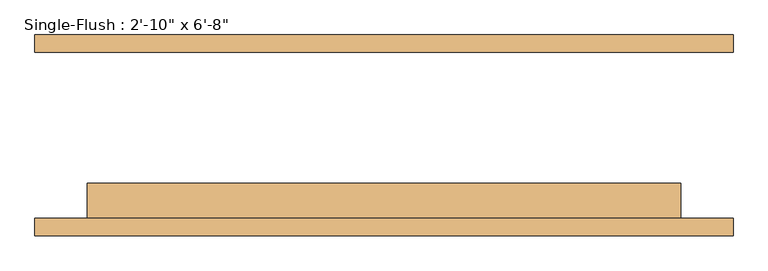
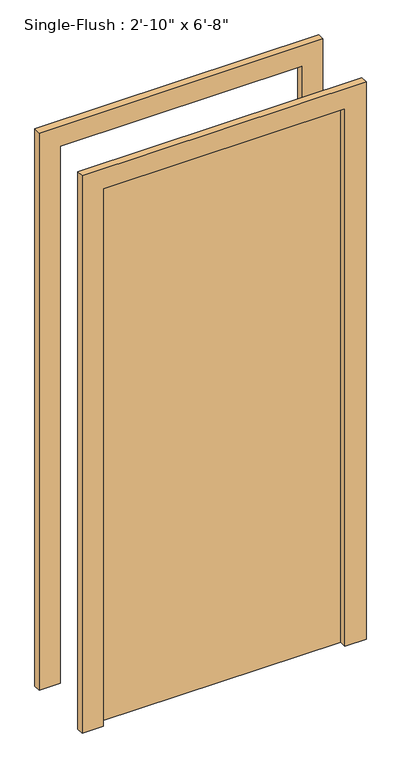
"""IFC4 building model written with IfcOpenShell, lengths in millimetres: door geometry."""

from ifc_helpers import new_model, si_unit, frame, origin, origin_with_axes, place, context, project, spatial, polyline, outline, extrude, source, transform, mapped, element, save


def door_8da58a41(model_context):
    return source(origin(), model_context, "Body", "SweptSolid", [
        extrude(outline(polyline([(2108.2, -508.0), (0.0, -508.0), (0.0, -431.8), (2032.0, -431.8), (2032.0, 431.8), (0.0, 431.8), (0.0, 508.0), (2108.2, 508.0), (2108.2, -508.0)])), frame((0.0, -146.05, 0.0), z_axis=(0.0, 1.0, 0.0), x_axis=(0.0, 0.0, 1.0)), (0.0, 0.0, 1.0), 25.4),
        extrude(outline(polyline([(2108.2, 508.0), (2108.2, -508.0), (0.0, -508.0), (0.0, -431.8), (2032.0, -431.8), (2032.0, 431.8), (0.0, 431.8), (0.0, 508.0), (2108.2, 508.0)])), frame((0.0, 120.65, 0.0), z_axis=(0.0, 1.0, 0.0), x_axis=(0.0, 0.0, 1.0)), (0.0, 0.0, 1.0), 25.4),
        extrude(outline(polyline([(431.8, -69.85), (431.8, -120.65), (-431.8, -120.65), (-431.8, -69.85), (431.8, -69.85)])), origin_with_axes(), (0.0, 0.0, 1.0), 2032.0),
    ])


if __name__ == "__main__":
    model = new_model("IFC4")
    model_context = context("Model", 3, world=origin())
    ifc_project = project(units=[si_unit("LENGTHUNIT", "METRE", prefix="MILLI")], contexts=[model_context])
    site = spatial("IfcSite", under=ifc_project)
    building = spatial("IfcBuilding", under=site)
    placement = place(None, origin())
    door_shape = door_8da58a41(model_context)
    element("IfcDoor", 1, ObjectType="Single-Flush : 2'-10\" x 6'-8\"", at=placement, inside=building, context=model_context, shape_type="MappedRepresentation", body=[
        mapped(door_shape, transform((0.0, 0.0, 0.0), x_axis=(1.0, 0.0, 0.0), y_axis=(0.0, 1.0, 0.0), z_axis=(0.0, 0.0, 1.0))),
    ])
    save(model, "model.ifc")

# Revit data of these elements
# Type "Single-Flush : 2'-10\" x 6'-8\""
#   Type Mark = "14"
#   Construction Type Id = "MDOOR"
#   Assembly Code = "C1020"
#   Analytic Construction = "Metal"
#   Thickness = 0' - 2"
#   Heat Transfer Coefficient (U) = 3.7021 W/(m²·K)
#   Height = 6' - 8"
#   Trim Projection Ext = 0' - 1"
#   Trim Projection Int = 0' - 1"
#   Trim Width = 0' - 3"
#   Width = 2' - 10"
#   Door Material = Door - Panel
#   Frame Material = Door - Frame
#   Visual Light Transmittance = 0
#   Solar Heat Gain Coefficient = 0
#   Function = (empty or 0)
#   Wall Closure = (empty or 0)
# Element 1 (IfcDoor, "Single-Flush : 2'-10\" x 6'-8\"")
#   Materials on its faces: "Door - Frame", "Door - Panel"
# Materials
#   "Door - Panel": class "Wood", colour RGB 210 159 95, transparency 0, Cost = 0
#   "Door - Frame": class "Miscellaneous", colour RGB 118 70 51, transparency 0, Cost = 0
